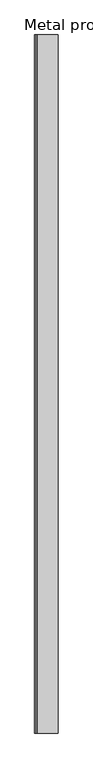
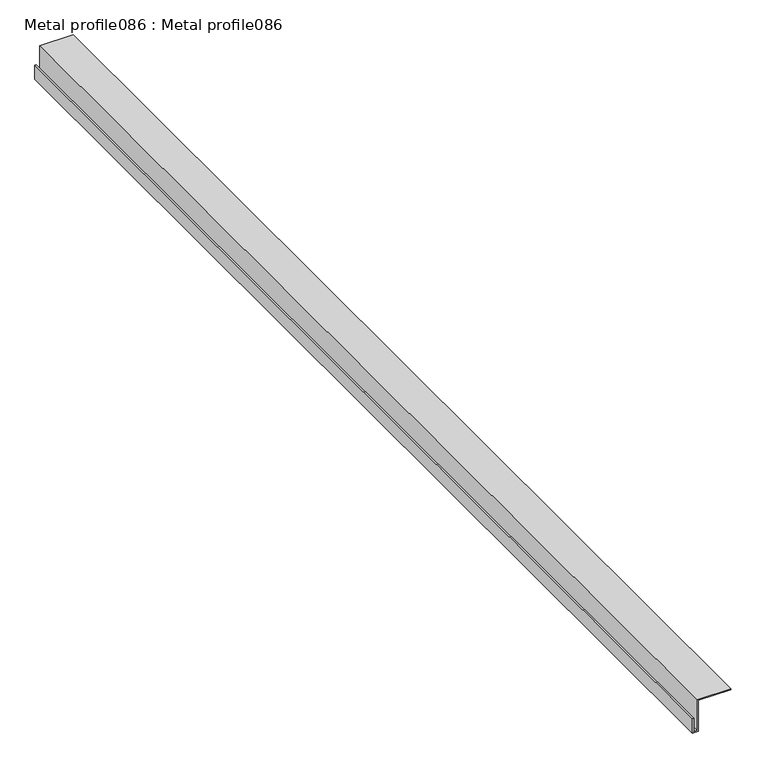
"""IFC4 building model written with IfcOpenShell, lengths in millimetres: proxy geometry, Metal profile086 : Metal profile086."""

from ifc_helpers import new_model, si_unit, frame, origin, place, context, project, spatial, polyline, outline, extrude, source, transform, mapped, element, save


def metal_profile086_metal_profile086_d3e08d76(model_context):
    return source(origin(), model_context, "Body", "SweptSolid", [
        extrude(outline(polyline([(42539.036776, -2413.4999158), (42539.036776, -2403.0365369), (42596.146151, -2403.0365369), (42596.146151, -2346.3602674), (42598.146151, -2346.3602674), (42598.146151, -2405.0365369), (42541.036776, -2405.0365369), (42541.036776, -2411.4999158), (42565.411776, -2411.4999158), (42565.411776, -2413.4999158), (42539.036776, -2413.4999158)])), frame((0.0, -1052.8906574, 0.0), z_axis=(0.0, 1.0, 0.0), x_axis=(0.0, 0.0, 1.0)), (0.0, 0.0, 1.0), 2000.0),
    ])


if __name__ == "__main__":
    model = new_model("IFC4")
    model_context = context("Model", 3, world=origin())
    ifc_project = project(units=[si_unit("LENGTHUNIT", "METRE", prefix="MILLI")], contexts=[model_context])
    site = spatial("IfcSite", under=ifc_project)
    building = spatial("IfcBuilding", under=site)
    placement = place(None, origin())
    metal_profile086_metal_profile086_shape = metal_profile086_metal_profile086_d3e08d76(model_context)
    element("IfcBuildingElementProxy", 1, Name="Metal profile086 : Metal profile086", ObjectType="Metal profile086 : Metal profile086", at=placement, inside=building, context=model_context, shape_type="MappedRepresentation", body=[
        mapped(metal_profile086_metal_profile086_shape, transform((0.0, 0.0, 0.0), x_axis=(1.0, 0.0, 0.0), y_axis=(0.0, 1.0, 0.0), z_axis=(0.0, 0.0, 1.0))),
    ])
    save(model, "model.ifc")

# Revit data of these elements
# Type "Metal profile086 : Metal profile086"
#   NameOverride = "Metal profile086"
# Element 1 (IfcBuildingElementProxy, "Metal profile086 : Metal profile086")
#   Materials on its faces: "ANGLE TRIM 1419"
# Materials
#   "ANGLE TRIM 1419": class "Unassigned", colour RGB 250 255 0, transparency 0
